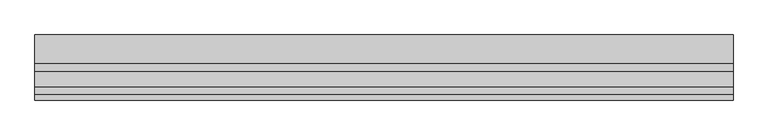
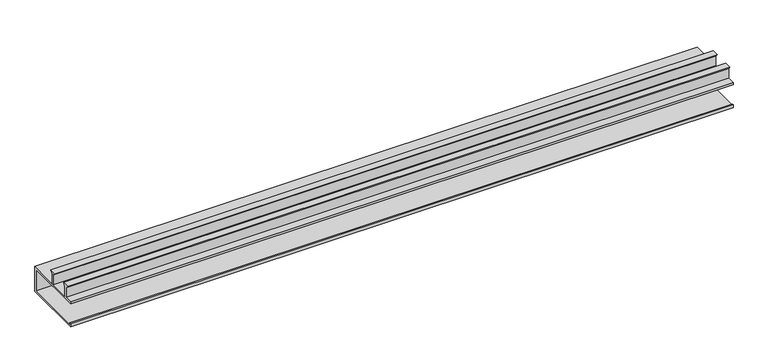
"""IFC4 building model written with IfcOpenShell, lengths in millimetres: proxy geometry, TN_ПВХ Гидрошпонка ТехноНИКОЛЬ FM_FMR : ПВХ Гидрошпонка ТехноНИКОЛЬ FMR-140/50."""

from ifc_helpers import new_model, si_unit, frame, origin, place, context, project, spatial, polyline, outline, extrude, source, transform, mapped, element, save


def specialty_equipment_6f71e63c(model_context):
    return source(origin(), model_context, "Body", "SweptSolid", [
        extrude(outline(polyline([(-5.0, 5.0), (-5.0, 55.0), (-140.0, 55.0), (-140.0, 60.0), (-122.1, 60.0), (-122.1, 83.120566), (-127.8725305, 90.0), (-112.1274695, 90.0), (-117.9, 83.120566), (-117.9, 60.0), (-72.1, 60.0), (-72.1, 83.120566), (-77.8725305, 90.0), (-62.1274695, 90.0), (-67.9, 83.120566), (-67.9, 60.0), (0.0, 60.0), (0.0, 0.0), (-140.0, 0.0), (-140.0, 7.5), (-137.0, 7.5), (-137.0, 5.0), (-5.0, 5.0)])), frame((0.0, 0.0, 0.0), z_axis=(1.0, 0.0, 0.0), x_axis=(0.0, 1.0, 0.0)), (0.0, 0.0, 1.0), 1500.0),
    ])


if __name__ == "__main__":
    model = new_model("IFC4")
    model_context = context("Model", 3, world=origin())
    ifc_project = project(units=[si_unit("LENGTHUNIT", "METRE", prefix="MILLI")], contexts=[model_context])
    site = spatial("IfcSite", under=ifc_project)
    building = spatial("IfcBuilding", under=site)
    placement = place(None, origin())
    specialty_equipment_shape = specialty_equipment_6f71e63c(model_context)
    element("IfcBuildingElementProxy", 1, Name="TN_ПВХ Гидрошпонка ТехноНИКОЛЬ FM_FMR : ПВХ Гидрошпонка ТехноНИКОЛЬ FMR-140/50", ObjectType="TN_ПВХ Гидрошпонка ТехноНИКОЛЬ FM_FMR : ПВХ Гидрошпонка ТехноНИКОЛЬ FMR-140/50", at=placement, inside=building, context=model_context, shape_type="MappedRepresentation", body=[
        mapped(specialty_equipment_shape, transform((0.0, 0.0, 0.0), x_axis=(1.0, 0.0, 0.0), y_axis=(0.0, 1.0, 0.0), z_axis=(0.0, 0.0, 1.0))),
    ])
    save(model, "model.ifc")

# Revit data of these elements
# Type "TN_ПВХ Гидрошпонка ТехноНИКОЛЬ FM_FMR : ПВХ Гидрошпонка ТехноНИКОЛЬ FMR-140/50"
#   Description = "Гидрошпонка для герметизации деформационных швов в монолитных железобетонных конструкциях заглубленных в грунт частей зданий, подземных сооружений (в том числе сооружений метрополитена), транспортных, железнодорожных и гидротехнических тоннелей. Применяется при сопряжении с существующими конструкциями или ранее возведенными конструкциями одного сооружения."
#   Type Comments = "п.м."
#   Manufacturer = "ТехноНИКОЛЬ"
#   ADSK_Примечание = ""
#   ADSK_Обозначение [instance default] = "ТехноНИКОЛЬ"
#   ADSK_Наименование = "ПВХ Гидрошпонка ТехноНИКОЛЬ FMR-140/50"
#   ADSK_Марка = ""
#   ADSK_Код изделия = "49886"
#   ADSK_Завод-изготовитель [instance default] = "ТехноНИКОЛЬ"
#   ADSK_Единица измерения [instance default] = "п.м."
#   ADSK_Группирование = "Гидрошпонки"
#   ADSK_URL страницы изделия = ""
#   ADSK_URL документации изделия = ""
#   built-in parameter 1001306 [instance default] = 3.28084 (stored number, unit not read)
#   ADSK_Размер_Длина [instance default] = 1000 mm
#   ADSK_Количество [instance default] = 1
#   ПВХ Гидрошпонка ТехноНИКОЛЬ FMR = yes
#   ПВХ Гидрошпонка ТехноНИКОЛЬ FM = no
#   Материал = TN_ПВХ_Черный
#   Default Elevation = 0
#   URL = ""
# Element 1 (IfcBuildingElementProxy, "TN_ПВХ Гидрошпонка ТехноНИКОЛЬ FM_FMR : ПВХ Гидрошпонка ТехноНИКОЛЬ FMR-140/50")
#   built-in parameter 1001306 = 4.92126 (stored number, unit not read)
#   ADSK_Размер_Длина = 1500 mm
#   ADSK_Количество = 1.5
#   Materials on its faces: "TN_ПВХ_Черный"
# Materials
#   "TN_ПВХ_Черный": class "Типовые", colour RGB 48 48 48, transparency 0, Cost = 0
